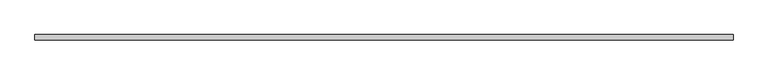
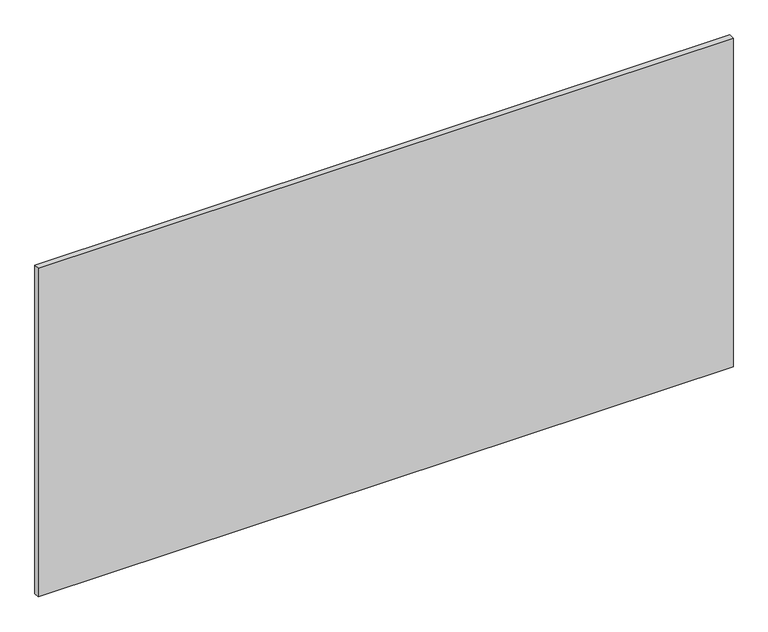
"""IFC4 building model written with IfcOpenShell, lengths in millimetres: proxy geometry, Inner panel:Inner panel:1:Inner panel:1 : Inner panel:Inner panel:300324:300043:Inner panel:1:Inner panel:1 : Inner panel:Inner panel:300324:300043 : Inner panel:Inner panel:1:Inner panel:1 : Inner panel:Inner panel:300324:300043:15 : Inner panel:Inner panel:1:Inner panel:1 : Inner panel:Inner panel:300324:300043:Inner panel:1:Inner panel:1 : Inner panel:Inner panel:300324:300043 : Inner panel:Inner panel:1:Inner panel:1 : Inner panel:Inner panel:300324:300043:300031."""

from ifc_helpers import new_model, si_unit, frame, origin, place, context, project, spatial, polyline, outline, extrude, source, transform, mapped, element, save


def generic_models_0ec44ed7(model_context):
    return source(origin(), model_context, "Body", "SweptSolid", [
        extrude(outline(polyline([(570452.6367239, -578778.4413841), (572891.0367239, -578778.4413841), (572891.0367239, -578797.4913841), (570452.6367239, -578797.4913841), (570452.6367239, -578778.4413841)])), frame((0.0, 0.0, 1270.0), z_axis=(0.0, 0.0, 1.0), x_axis=(1.0, 0.0, 0.0)), (0.0, 0.0, 1.0), 1219.2),
    ])


if __name__ == "__main__":
    model = new_model("IFC4")
    model_context = context("Model", 3, world=origin())
    ifc_project = project(units=[si_unit("LENGTHUNIT", "METRE", prefix="MILLI")], contexts=[model_context])
    site = spatial("IfcSite", under=ifc_project)
    building = spatial("IfcBuilding", under=site)
    placement = place(None, origin())
    generic_models_shape = generic_models_0ec44ed7(model_context)
    element("IfcBuildingElementProxy", 1, Name="Inner panel:Inner panel:1:Inner panel:1 : Inner panel:Inner panel:300324:300043:Inner panel:1:Inner panel:1 : Inner panel:Inner panel:300324:300043 : Inner panel:Inner panel:1:Inner panel:1 : Inner panel:Inner panel:300324:300043:15 : Inner panel:Inner panel:1:Inner panel:1 : Inner panel:Inner panel:300324:300043:Inner panel:1:Inner panel:1 : Inner panel:Inner panel:300324:300043 : Inner panel:Inner panel:1:Inner panel:1 : Inner panel:Inner panel:300324:300043:300031", ObjectType="Inner panel:Inner panel:1:Inner panel:1 : Inner panel:Inner panel:300324:300043:Inner panel:1:Inner panel:1 : Inner panel:Inner panel:300324:300043 : Inner panel:Inner panel:1:Inner panel:1 : Inner panel:Inner panel:300324:300043:15 : Inner panel:Inner panel:1:Inner panel:1 : Inner panel:Inner panel:300324:300043:Inner panel:1:Inner panel:1 : Inner panel:Inner panel:300324:300043 : Inner panel:Inner panel:1:Inner panel:1 : Inner panel:Inner panel:300324:300043:300031", at=placement, inside=building, context=model_context, shape_type="MappedRepresentation", body=[
        mapped(generic_models_shape, transform((0.0, 0.0, 0.0), x_axis=(1.0, 0.0, 0.0), y_axis=(0.0, 1.0, 0.0), z_axis=(0.0, 0.0, 1.0))),
    ])
    save(model, "model.ifc")

# Revit data of these elements
# Type "Inner panel:Inner panel:1:Inner panel:1 : Inner panel:Inner panel:300324:300043:Inner panel:1:Inner panel:1 : Inner panel:Inner panel:300324:300043 : Inner panel:Inner panel:1:Inner panel:1 : Inner panel:Inner panel:300324:300043:15 : Inner panel:Inner panel:1:Inner panel:1 : Inner panel:Inner panel:300324:300043:Inner panel:1:Inner panel:1 : Inner panel:Inner panel:300324:300043 : Inner panel:Inner panel:1:Inner panel:1 : Inner panel:Inner panel:300324:300043:300031"
#   NameOverride = "Inner panel:Inner panel:1:Inner panel:1 : Inner panel:Inner panel:300324:300043:Inner panel:1:Inner panel:1 : Inner panel:Inner panel:300324:300043 : Inner panel:Inner panel:1:Inner panel:1 : Inner panel:Inner panel:300324:300043:300031"
#   ObjectTypeOverride = "Inner panel:1:Inner panel:1 : Inner panel:Inner panel:300324:300043 : Inner panel:Inner panel:1:Inner panel:1 : Inner panel:Inner panel:300324:300043"
#   Reference = "Inner panel"
#   Tag = "300031"
# Element 1 (IfcBuildingElementProxy, "Inner panel:Inner panel:1:Inner panel:1 : Inner panel:Inner panel:300324:300043:Inner panel:1:Inner panel:1 : Inner panel:Inner panel:300324:300043 : Inner panel:Inner panel:1:Inner panel:1 : Inner panel:Inner panel:300324:300043:15 : Inner panel:Inner panel:1:Inner panel:1 : Inner panel:Inner panel:300324:300043:Inner panel:1:Inner panel:1 : Inner panel:Inner panel:300324:300043 : Inner panel:Inner panel:1:Inner panel:1 : Inner panel:Inner panel:300324:300043:300031")
#   Materials on its faces: "¾” (CLASS A) FIRE RETARDANT PLYWOOD ...OR… IF 1/4\" GYP. BD UNDER PLYWOOD, FLAME SPREAD TO BE CLASS C -  (FINISH: GRADE B - PREFINISHED STAINED/SEALED) - 1/4\" GAP BTWN PANELS (FASTENERS T.B.D.)"
# Materials
#   "¾” (CLASS A) FIRE RETARDANT PLYWOOD ...OR… IF 1/4\" GYP. BD UNDER PLYWOOD, FLAME SPREAD TO BE CLASS C -  (FINISH: GRADE B - PREFINISHED STAINED/SEALED) - 1/4\" GAP BTWN PANELS (FASTENERS T.B.D.)": class "Wood", colour RGB 149 120 74, transparency 0, Description = "Plywood, sheathing grade", Cost = 0
